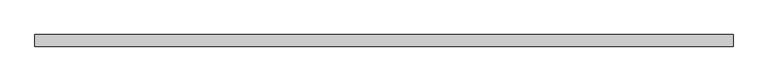
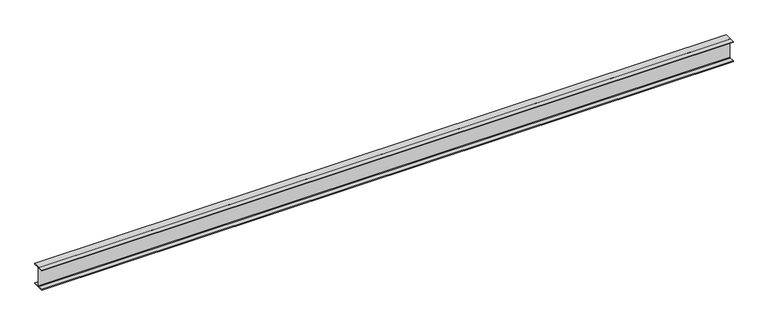
"""IFC4 building model written with IfcOpenShell, lengths in millimetres: beam geometry, Old_Steel Beam_H-KSD3502 : H_SB_ASB_H-488×300x11x18."""

from ifc_helpers import new_model, si_unit, point, frame, frame_2d, origin, place, context, project, spatial, polyline, circle_curve, trimmed, segment, composite_curve, outline, extrude, source, transform, mapped, element, save


def beam_7f8595ab(model_context):
    return source(origin(), model_context, "Body", "SweptSolid", [
        extrude(outline(composite_curve([segment(polyline([(82.5, -141.5), (82.5, -151.7), (-82.5, -151.7), (-82.5, -141.5), (-11.9, -141.5)]), True, "CONTINUOUS"), segment(trimmed(circle_curve(frame_2d((-11.9, -132.6)), 8.9), [point((-11.9, -141.5))], [point((-3.0, -132.6))], True, "CARTESIAN"), True, "CONTINUOUS"), segment(polyline([(-3.0, -132.6), (-3.0, 132.6)]), True, "CONTINUOUS"), segment(trimmed(circle_curve(frame_2d((-11.9, 132.6)), 8.9), [point((-3.0, 132.6))], [point((-11.9, 141.5))], True, "CARTESIAN"), True, "CONTINUOUS"), segment(polyline([(-11.9, 141.5), (-82.5, 141.5), (-82.5, 151.7), (82.5, 151.7), (82.5, 141.5), (11.9, 141.5)]), True, "CONTINUOUS"), segment(trimmed(circle_curve(frame_2d((11.9, 132.6)), 8.9), [point((11.9, 141.5))], [point((3.0, 132.6))], True, "CARTESIAN"), True, "CONTINUOUS"), segment(polyline([(3.0, 132.6), (3.0, -132.6)]), True, "CONTINUOUS"), segment(trimmed(circle_curve(frame_2d((11.9, -132.6)), 8.9), [point((3.0, -132.6))], [point((11.9, -141.5))], True, "CARTESIAN"), True, "CONTINUOUS"), segment(polyline([(11.9, -141.5), (82.5, -141.5)]), True, "CONTINUOUS")], self_intersect=False)), frame((-4962.3, 0.0, 0.0), z_axis=(1.0, 0.0, 0.0), x_axis=(0.0, 1.0, 0.0)), (0.0, 0.0, 1.0), 9924.6),
    ])


if __name__ == "__main__":
    model = new_model("IFC4")
    model_context = context("Model", 3, world=origin())
    ifc_project = project(units=[si_unit("LENGTHUNIT", "METRE", prefix="MILLI")], contexts=[model_context])
    site = spatial("IfcSite", under=ifc_project)
    building = spatial("IfcBuilding", under=site)
    placement = place(None, origin())
    beam_shape = beam_7f8595ab(model_context)
    element("IfcBeam", 1, ObjectType="Old_Steel Beam_H-KSD3502 : H_SB_ASB_H-488×300x11x18", at=placement, inside=building, context=model_context, shape_type="MappedRepresentation", body=[
        mapped(beam_shape, transform((0.0, 0.0, 0.0), x_axis=(1.0, 0.0, 0.0), y_axis=(0.0, 1.0, 0.0), z_axis=(0.0, 0.0, 1.0))),
    ])
    save(model, "model.ifc")

# Revit data of these elements
# Type "Old_Steel Beam_H-KSD3502 : H_SB_ASB_H-488×300x11x18"
#   Width = 30.0 cm
#   Web Thickness = 1.1 cm
#   Web Fillet = 2.6 cm
#   Warping Constant = 4473230.0 cm⁶
#   Torsional Moment of Inertia = 137.492 cm⁴
#   Torsional Modulus = 1.0 cm³
#   Section Area = 163.5 cm²
#   Plastic Modulus weak axis = 830.0 cm³
#   Plastic Modulus strong axis = 3230.0 cm³
#   Perimeter = 2.11 m²/m
#   Nominal Weight = 128.00 kgf/m
#   Moment of Inertia weak axis = 8110.00 cm⁴
#   Moment of Inertia strong axis = 71000.00 cm⁴
#   Height = 48.8 cm
#   Flange Thickness = 1.8 cm
#   Elastic Modulus weak axis = 541.0 cm³
#   Elastic Modulus strong axis = 2910.0 cm³
#   Centroid Vertical = 24.4 cm
#   Centroid Horizontal = 15.0 cm
#   Length [instance default] = 1.5240 m
#   Structural Material [instance default] = Steel, 45-345
#   Assembly Code = ""
# Element 1 (IfcBeam, "Old_Steel Beam_H-KSD3502 : H_SB_ASB_H-488×300x11x18")
#   Structural Material = none
# Materials
#   "Steel, 45-345": class "Metal", colour RGB 189 187 185, transparency 0, Description = "Steel 345 MPa", Cost = 0
